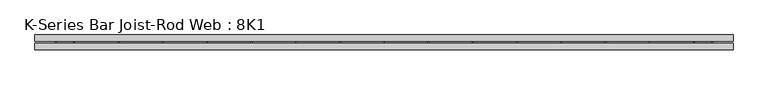
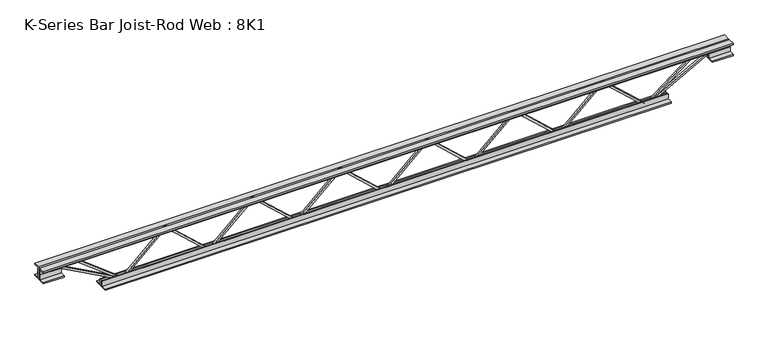
"""IFC4 building model written with IfcOpenShell, lengths in millimetres: beam geometry, K-Series Bar Joist-Rod Web : 8K1."""

from ifc_helpers import new_model, si_unit, frame, origin, place, context, project, spatial, polyline, outline, extrude, source, transform, mapped, element, save


def k_series_bar_joist_rod_web_8k1_7ca94746(model_context):
    return source(origin(), model_context, "Body", "SweptSolid", [
        extrude(outline(polyline([(-90.4875, 430.0376473), (-100.0125, 430.0376473), (-100.0125, 435.059607), (90.4875, 643.7284306), (90.4875, 646.3845111), (-100.0125, 855.0533348), (-100.0125, 860.0752945), (-90.4875, 860.0752945), (-90.4875, 858.7472543), (100.0125, 650.0784306), (100.0125, 640.0345111), (-90.4875, 431.3656875), (-90.4875, 430.0376473)])), frame((0.0, -4.7625, 0.0), z_axis=(0.0, 1.0, 0.0), x_axis=(0.0, 0.0, 1.0)), (0.0, 0.0, 1.0), 9.525),
        extrude(outline(polyline([(-90.4875, 0.0), (-100.0125, 0.0), (-100.0125, 5.0219598), (90.4875, 213.6907834), (90.4875, 216.3468639), (-100.0125, 425.0156875), (-100.0125, 430.0376473), (-90.4875, 430.0376473), (-90.4875, 428.709607), (100.0125, 220.0407834), (100.0125, 209.9968639), (-90.4875, 1.3280402), (-90.4875, 0.0)])), frame((0.0, -4.7625, 0.0), z_axis=(0.0, 1.0, 0.0), x_axis=(0.0, 0.0, 1.0)), (0.0, 0.0, 1.0), 9.525),
        extrude(outline(polyline([(-90.4875, -430.0376473), (-100.0125, -430.0376473), (-100.0125, -425.0156875), (90.4875, -216.3468639), (90.4875, -213.6907834), (-100.0125, -5.0219598), (-100.0125, 0.0), (-90.4875, 0.0), (-90.4875, -1.3280402), (100.0125, -209.9968639), (100.0125, -220.0407834), (-90.4875, -428.709607), (-90.4875, -430.0376473)])), frame((0.0, -4.7625, 0.0), z_axis=(0.0, 1.0, 0.0), x_axis=(0.0, 0.0, 1.0)), (0.0, 0.0, 1.0), 9.525),
        extrude(outline(polyline([(-90.4875, -860.0752945), (-100.0125, -860.0752945), (-100.0125, -855.0533348), (90.4875, -646.3845111), (90.4875, -643.7284306), (-100.0125, -435.059607), (-100.0125, -430.0376473), (-90.4875, -430.0376473), (-90.4875, -431.3656875), (100.0125, -640.0345111), (100.0125, -650.0784306), (-90.4875, -858.7472543), (-90.4875, -860.0752945)])), frame((0.0, -4.7625, 0.0), z_axis=(0.0, 1.0, 0.0), x_axis=(0.0, 0.0, 1.0)), (0.0, 0.0, 1.0), 9.525),
        extrude(outline(polyline([(-90.4875, 860.0752945), (-100.0125, 860.0752945), (-100.0125, 865.0972543), (90.4875, 1073.7660779), (90.4875, 1076.4221584), (-100.0125, 1285.090982), (-100.0125, 1290.1129418), (-90.4875, 1290.1129418), (-90.4875, 1288.7849015), (100.0125, 1080.1160779), (100.0125, 1070.0721584), (-90.4875, 861.4033348), (-90.4875, 860.0752945)])), frame((0.0, -4.7625, 0.0), z_axis=(0.0, 1.0, 0.0), x_axis=(0.0, 0.0, 1.0)), (0.0, 0.0, 1.0), 9.525),
        extrude(outline(polyline([(-90.4875, -1290.1129418), (-100.0125, -1290.1129418), (-100.0125, -1285.090982), (90.4875, -1076.4221584), (90.4875, -1073.7660779), (-100.0125, -865.0972543), (-100.0125, -860.0752945), (-90.4875, -860.0752945), (-90.4875, -861.4033348), (100.0125, -1070.0721584), (100.0125, -1080.1160779), (-90.4875, -1288.7849015), (-90.4875, -1290.1129418)])), frame((0.0, -4.7625, 0.0), z_axis=(0.0, 1.0, 0.0), x_axis=(0.0, 0.0, 1.0)), (0.0, 0.0, 1.0), 9.525),
        extrude(outline(polyline([(4.7625, 101.6), (36.5125, 101.6), (36.5125, 95.25), (11.1125, 95.25), (11.1125, 69.85), (4.7625, 69.85), (4.7625, 101.6)])), frame((-1696.5129418, 0.0, 0.0), z_axis=(1.0, 0.0, 0.0), x_axis=(0.0, 1.0, 0.0)), (0.0, 0.0, 1.0), 3393.0258836),
        extrude(outline(polyline([(-4.7625, 101.6), (-4.7625, 69.85), (-11.1125, 69.85), (-11.1125, 95.25), (-36.5125, 95.25), (-36.5125, 101.6), (-4.7625, 101.6)])), frame((-1696.5129418, 0.0, 0.0), z_axis=(1.0, 0.0, 0.0), x_axis=(0.0, 1.0, 0.0)), (0.0, 0.0, 1.0), 3393.0258836),
        extrude(outline(polyline([(-4.7625, 38.1), (-36.5125, 38.1), (-36.5125, 44.45), (-11.1125, 44.45), (-11.1125, 69.85), (-4.7625, 69.85), (-4.7625, 38.1)])), frame((-1696.5129418, 0.0, 0.0), z_axis=(1.0, 0.0, 0.0), x_axis=(0.0, 1.0, 0.0)), (0.0, 0.0, 1.0), 101.6),
        extrude(outline(polyline([(36.5125, 38.1), (4.7625, 38.1), (4.7625, 69.85), (11.1125, 69.85), (11.1125, 44.45), (36.5125, 44.45), (36.5125, 38.1)])), frame((-1696.5129418, 0.0, 0.0), z_axis=(1.0, 0.0, 0.0), x_axis=(0.0, 1.0, 0.0)), (0.0, 0.0, 1.0), 101.6),
        extrude(outline(polyline([(4.7625, 38.1), (4.7625, 69.85), (11.1125, 69.85), (11.1125, 44.45), (36.5125, 44.45), (36.5125, 38.1), (4.7625, 38.1)])), frame((1594.9129418, 0.0, 0.0), z_axis=(1.0, 0.0, 0.0), x_axis=(0.0, 1.0, 0.0)), (0.0, 0.0, 1.0), 101.6),
        extrude(outline(polyline([(-4.7625, 38.1), (-36.5125, 38.1), (-36.5125, 44.45), (-11.1125, 44.45), (-11.1125, 69.85), (-4.7625, 69.85), (-4.7625, 38.1)])), frame((1594.9129418, 0.0, 0.0), z_axis=(1.0, 0.0, 0.0), x_axis=(0.0, 1.0, 0.0)), (0.0, 0.0, 1.0), 101.6),
        extrude(outline(polyline([(4.7625, -101.6), (4.7625, -69.85), (11.1125, -69.85), (11.1125, -95.25), (36.5125, -95.25), (36.5125, -101.6), (4.7625, -101.6)])), frame((-1391.7129418, 0.0, 0.0), z_axis=(1.0, 0.0, 0.0), x_axis=(0.0, 1.0, 0.0)), (0.0, 0.0, 1.0), 2783.4258836),
        extrude(outline(polyline([(-4.7625, -101.6), (-36.5125, -101.6), (-36.5125, -95.25), (-11.1125, -95.25), (-11.1125, -69.85), (-4.7625, -69.85), (-4.7625, -101.6)])), frame((-1391.7129418, 0.0, 0.0), z_axis=(1.0, 0.0, 0.0), x_axis=(0.0, 1.0, 0.0)), (0.0, 0.0, 1.0), 2783.4258836),
        extrude(outline(polyline([(0.0, -9.525), (0.0, 0.0), (346.6425392, 0.0), (346.6425392, -9.525), (0.0, -9.525)])), frame((-1597.1812403, 4.7625, 65.662372), z_axis=(0.47628314854008014, 0.0, 0.8792919665371384), x_axis=(0.8792919665371384, 0.0, -0.47628314854008014)), (0.0, 0.0, 1.0), 9.525),
        extrude(outline(polyline([(0.0, -9.525), (0.0, 0.0), (271.092428, 0.0), (271.092428, -9.525), (0.0, -9.525)])), frame((-1508.0322107, 4.7625, 66.0725904), z_axis=(0.6090173791345892, 0.0, 0.793156877239324), x_axis=(0.793156877239324, 0.0, -0.6090173791345892)), (0.0, 0.0, 1.0), 9.525),
        extrude(outline(polyline([(0.0, -9.525), (0.0, 0.0), (346.6425392, 0.0), (346.6425392, -9.525), (0.0, -9.525)])), frame((1597.1812403, -4.7625, 65.662372), z_axis=(-0.47628314854004167, 0.0, 0.8792919665371591), x_axis=(-0.8792919665371591, 0.0, -0.47628314854004167)), (0.0, 0.0, 1.0), 9.525),
        extrude(outline(polyline([(0.0, -9.525), (0.0, 0.0), (271.092428, 0.0), (271.092428, -9.525), (0.0, -9.525)])), frame((1508.0322107, -4.7625, 66.0725904), z_axis=(-0.6090173791345677, 0.0, 0.7931568772393406), x_axis=(-0.7931568772393406, 0.0, -0.6090173791345677)), (0.0, 0.0, 1.0), 9.525),
    ])


if __name__ == "__main__":
    model = new_model("IFC4")
    model_context = context("Model", 3, world=origin())
    ifc_project = project(units=[si_unit("LENGTHUNIT", "METRE", prefix="MILLI")], contexts=[model_context])
    site = spatial("IfcSite", under=ifc_project)
    building = spatial("IfcBuilding", under=site)
    placement = place(None, origin())
    k_series_bar_joist_rod_web_8k1_shape = k_series_bar_joist_rod_web_8k1_7ca94746(model_context)
    element("IfcBeam", 1, ObjectType="K-Series Bar Joist-Rod Web : 8K1", at=placement, inside=building, context=model_context, shape_type="MappedRepresentation", body=[
        mapped(k_series_bar_joist_rod_web_8k1_shape, transform((0.0, 0.0, 0.0), x_axis=(1.0, 0.0, 0.0), y_axis=(0.0, 1.0, 0.0), z_axis=(0.0, 0.0, 1.0))),
    ])
    save(model, "model.ifc")

# Revit data of these elements
# Type "K-Series Bar Joist-Rod Web : 8K1"
#   Assembly Code = "B1010350"
#   Wt = 5.1
#   Web Thickness = 0' - 0 3/8"
#   Start Offset [instance default] = 0' - 0"
#   Start Extension [instance default] = 0' - 0"
#   Seat Length = 0' - 4"
#   Seat Depth = 0' - 2 1/2"
#   PanelArrayLength [instance default] = 21' - 4"
#   Panel [instance default] = 1' - 4"
#   End Offset [instance default] = 0' - 0"
#   End Extension [instance default] = 0' - 0"
#   End Panel = 1' - 4"
#   Cord Leg = 0' - 1 1/4"
#   Chord Thickness = 0' - 0 1/4"
#   Length [instance default] = 24' - 0"
#   Depth = 0' - 8"
#   PanelArrayNum [instance default] = 16
#   Rendering Material = none
# Element 1 (IfcBeam, "K-Series Bar Joist-Rod Web : 8K1")
#   PanelArrayLength = 8' - 5.5837"
#   Panel = 1' - 4.93062"
#   PanelArrayNum = 6
